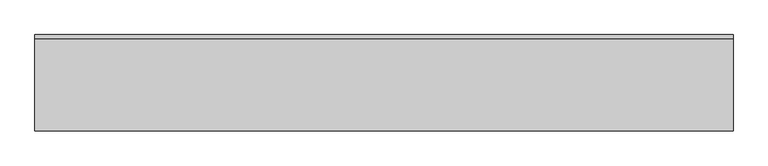
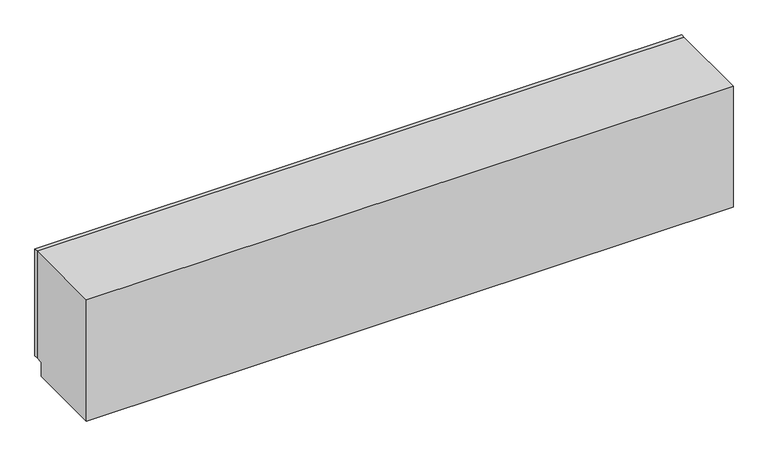
"""IFC4 building model written with IfcOpenShell, lengths in millimetres: furniture geometry, OD_CW_Base Cabinet : OD_CW_Base Cabinet."""

from ifc_helpers import new_model, si_unit, frame, origin, place, context, project, spatial, polyline, outline, extrude, source, transform, mapped, element, save


def furniture_41a9c5b6(model_context):
    return source(origin(), model_context, "Body", "SweptSolid", [
        extrude(outline(polyline([(18.7377049, -25.4), (18.7377049, 0.0), (4438.3377049, 0.0), (4438.3377049, -25.4), (18.7377049, -25.4)])), frame((0.0, 0.0, 101.6), z_axis=(0.0, 0.0, 1.0), x_axis=(1.0, 0.0, 0.0)), (0.0, 0.0, 1.0), 774.7),
        extrude(outline(polyline([(-25.4, 876.3), (-25.4, 101.6), (-76.2, 101.6), (-76.2, 0.0), (-609.6, 0.0), (-609.6, 876.3), (-25.4, 876.3)])), frame((18.7377049, 0.0, 0.0), z_axis=(1.0, 0.0, 0.0), x_axis=(0.0, 1.0, 0.0)), (0.0, 0.0, 1.0), 4419.6),
    ])


if __name__ == "__main__":
    model = new_model("IFC4")
    model_context = context("Model", 3, world=origin())
    ifc_project = project(units=[si_unit("LENGTHUNIT", "METRE", prefix="MILLI")], contexts=[model_context])
    site = spatial("IfcSite", under=ifc_project)
    building = spatial("IfcBuilding", under=site)
    placement = place(None, origin())
    furniture_shape = furniture_41a9c5b6(model_context)
    element("IfcFurniture", 1, ObjectType="OD_CW_Base Cabinet : OD_CW_Base Cabinet", at=placement, inside=building, context=model_context, shape_type="MappedRepresentation", body=[
        mapped(furniture_shape, transform((0.0, 0.0, 0.0), x_axis=(1.0, 0.0, 0.0), y_axis=(0.0, 1.0, 0.0), z_axis=(0.0, 0.0, 1.0))),
    ])
    save(model, "model.ifc")

# Revit data of these elements
# Type "OD_CW_Base Cabinet : OD_CW_Base Cabinet"
#   OD_CW_Width [instance default] = 2' - 10"
#   OD_CW_Length [instance default] = 8' - 0"
#   OD_CW_Height [instance default] = 2' - 3"
#   Depth = 2' - 0"
#   Height = 3' - 0"
#   Width = 4' - 0"
#   OD_CW_Material_Front Panel [instance default] = none
#   OD_CW_Material_Body [instance default] = none
# Element 1 (IfcFurniture, "OD_CW_Base Cabinet : OD_CW_Base Cabinet")
#   OD_CW_Width = 2' - 0"
#   OD_CW_Length = 14' - 6"
#   OD_CW_Height = 2' - 10 1/2"
#   Materials on its faces: "CASEWORK"
# Materials
#   "CASEWORK": class "Generic", colour RGB 181 181 181, transparency 0, Cost = 0
